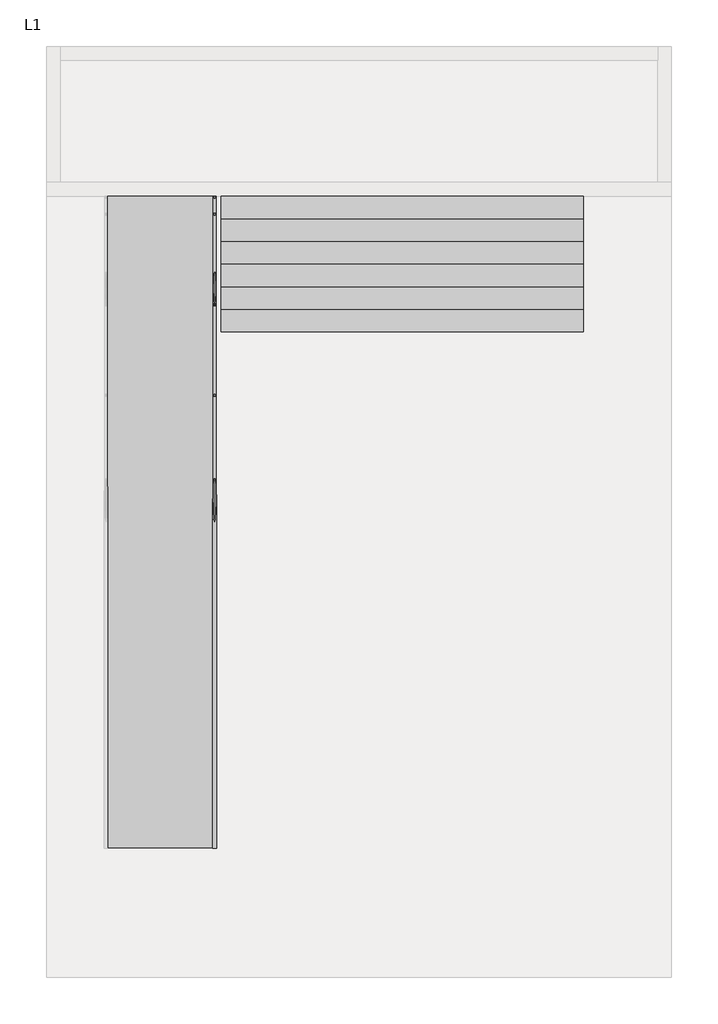
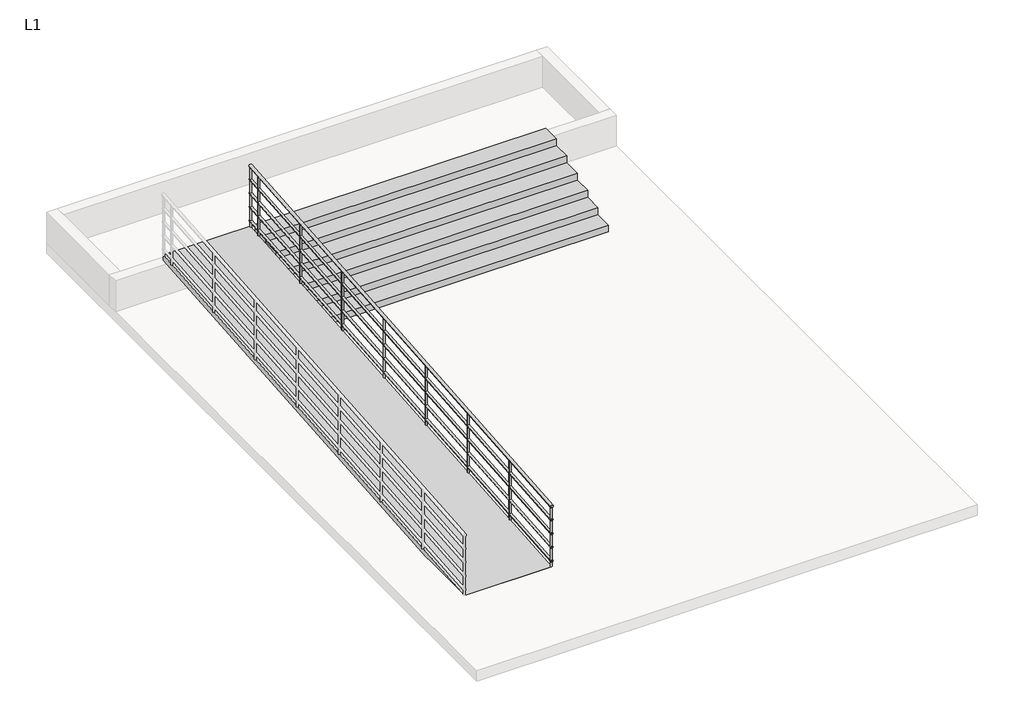
# One storey, part 2 of 2: 1 railing, 1 ramp, 1 stair flight.
"""IFC4 building model written with IfcOpenShell, lengths in millimetres."""

import ifcopenshell
import ifcopenshell.guid

model = None  # the IFC model being written
_history = None  # IfcOwnerHistory: only IFC2X3 demands one
_inside = {}  # id of a spatial element -> (the spatial element, [elements in it])
_under = {}  # id of a project, library or spatial element -> (it, [spatial elements below it])
_declared = {}  # id of a project -> (the project, [libraries it declares])
_typed = {}  # id of a type object -> (the type object, [elements of that type])
_made_of = {}  # id of a material, layer set ... -> (it, [elements and type objects made of it])


def new_model(schema):
    """Start an empty IFC model of exactly this schema.

    Asked for "IFC4X3", IfcOpenShell would pick the latest addendum, in which some entities
    have other attributes; the version numbers below select the first issue.
    IFC2X3 requires an IfcOwnerHistory on every rooted entity: one is made here for all.
    """
    global model, _history
    if schema == "IFC4X3":
        model = ifcopenshell.file(schema_version=(4, 3, 0, 0))
    else:
        model = ifcopenshell.file(schema=schema)
    _inside.clear()
    _under.clear()
    _declared.clear()
    _typed.clear()
    _made_of.clear()
    _history = None
    if model.schema == "IFC2X3":
        org = make("IfcOrganization", Name="unknown")
        user = make(
            "IfcPersonAndOrganization",
            ThePerson=make("IfcPerson", FamilyName="unknown"),
            TheOrganization=org,
        )
        app = make(
            "IfcApplication",
            ApplicationDeveloper=org,
            Version="unknown",
            ApplicationFullName="unknown",
            ApplicationIdentifier="unknown",
        )
        _history = make(
            "IfcOwnerHistory",
            OwningUser=user,
            OwningApplication=app,
            ChangeAction="ADDED",
            CreationDate=0,
        )
    return model


def make(cls, **values):
    """One entity of the class cls with the attributes given. An attribute that is None is left unset."""
    return model.create_entity(
        cls, **{name: value for name, value in values.items() if value is not None}
    )


def rooted(cls, **values):
    """An entity with a GlobalId (a new one), such as an element, a storey or a relation."""
    return make(cls, GlobalId=ifcopenshell.guid.new(), OwnerHistory=_history, **values)


def si_unit(unit_type, name, prefix=None):
    """IfcSIUnit, for example si_unit("LENGTHUNIT", "METRE", prefix="MILLI")."""
    return make("IfcSIUnit", UnitType=unit_type, Prefix=prefix, Name=name)


def assignment(units):
    """IfcUnitAssignment: the units of a project."""
    return None if units is None else make("IfcUnitAssignment", Units=units)


def point(xyz):
    """IfcCartesianPoint."""
    return None if xyz is None else make("IfcCartesianPoint", Coordinates=xyz)


def direction(xyz):
    """IfcDirection."""
    return None if xyz is None else make("IfcDirection", DirectionRatios=xyz)


def frame(location, z_axis=None, x_axis=None):
    """IfcAxis2Placement3D, a coordinate frame: its origin and axes. An axis left out is left unset."""
    return make(
        "IfcAxis2Placement3D",
        Location=point(location),
        Axis=direction(z_axis),
        RefDirection=direction(x_axis),
    )


def origin():
    """The frame at (0, 0, 0) with its axes left unset."""
    return frame((0.0, 0.0, 0.0))


def place(relative_to, where):
    """IfcLocalPlacement: puts the frame where relative to a parent placement (None: the world)."""
    return make(
        "IfcLocalPlacement", PlacementRelTo=relative_to, RelativePlacement=where
    )


def context(
    kind, dimensions, precision=None, world=None, true_north=None, identifier=None
):
    """IfcGeometricRepresentationContext, for example the 3D "Model" context."""
    return make(
        "IfcGeometricRepresentationContext",
        ContextIdentifier=identifier,
        ContextType=kind,
        CoordinateSpaceDimension=dimensions,
        Precision=precision,
        WorldCoordinateSystem=world,
        TrueNorth=true_north,
    )


def project(units=None, contexts=None):
    """IfcProject with its units and contexts."""
    return rooted(
        "IfcProject",
        Name="project",
        RepresentationContexts=contexts,
        UnitsInContext=assignment(units),
    )


def spatial(cls, under=None, at=None, **own):
    """A site, building, storey or space (cls), placed at a placement, below another one or the project."""
    s = rooted(cls, ObjectPlacement=at, **own)
    if under is not None:
        _under.setdefault(under.id(), (under, []))[1].append(s)
    return s


def polyline(points):
    """IfcPolyline through the points."""
    return make("IfcPolyline", Points=[point(p) for p in points])


def ellipse_curve(where, semi_axis1, semi_axis2):
    """IfcEllipse in the frame where."""
    return make(
        "IfcEllipse", Position=where, SemiAxis1=semi_axis1, SemiAxis2=semi_axis2
    )


def outline(outer, holes=None, kind="AREA"):
    """IfcArbitraryClosedProfileDef: a profile drawn as a closed curve; with holes, ...WithVoids."""
    if holes is None:
        return make("IfcArbitraryClosedProfileDef", ProfileType=kind, OuterCurve=outer)
    return make(
        "IfcArbitraryProfileDefWithVoids",
        ProfileType=kind,
        OuterCurve=outer,
        InnerCurves=holes,
    )


def extrude(swept, where, along, depth):
    """IfcExtrudedAreaSolid: the profile swept, set in the frame where, extruded along a direction by depth."""
    return make(
        "IfcExtrudedAreaSolid",
        SweptArea=swept,
        Position=where,
        ExtrudedDirection=direction(along),
        Depth=depth,
    )


def faces_of(points, faces, orient=None, outer=None):
    """IfcFace entities. A face is a list of loops; a loop is a list of indices into points, from 0.

    orient and outer hold one flag for each loop. By default every Orientation is true, the
    first loop of a face is its IfcFaceOuterBound and the others are IfcFaceBound.
    """
    made = []
    for i, loops in enumerate(faces):
        bounds = []
        for j, loop in enumerate(loops):
            is_outer = j == 0 if outer is None else outer[i][j]
            bounds.append(
                make(
                    "IfcFaceOuterBound" if is_outer else "IfcFaceBound",
                    Bound=make("IfcPolyLoop", Polygon=[points[k] for k in loop]),
                    Orientation=True if orient is None else orient[i][j],
                )
            )
        made.append(make("IfcFace", Bounds=bounds))
    return made


def faceted_brep(points, faces, orient=None, outer=None, voids=None):
    """IfcFacetedBrep: a solid bounded by flat faces; with voids (closed shells), ...WithVoids."""
    shared = [point(p) for p in points]
    hull = make("IfcClosedShell", CfsFaces=faces_of(shared, faces, orient, outer))
    if voids is None:
        return make("IfcFacetedBrep", Outer=hull)
    return make(
        "IfcFacetedBrepWithVoids",
        Outer=hull,
        Voids=[
            make(cls, CfsFaces=faces_of(shared, fs, o, b)) for cls, fs, o, b in voids
        ],
    )


def shape(context_of_items, identifier, shape_type, items):
    """IfcShapeRepresentation: the items that make up one representation, for example the "Body"."""
    return make(
        "IfcShapeRepresentation",
        ContextOfItems=context_of_items,
        RepresentationIdentifier=identifier,
        RepresentationType=shape_type,
        Items=items,
    )


def source(mapping_origin, context_of_items, identifier, shape_type, items):
    """IfcRepresentationMap: a shape defined once, which mapped items show again and again."""
    return make(
        "IfcRepresentationMap",
        MappingOrigin=mapping_origin,
        MappedRepresentation=shape(context_of_items, identifier, shape_type, items),
    )


def transform(
    local_origin,
    x_axis=None,
    y_axis=None,
    z_axis=None,
    scale=None,
    scale2=None,
    scale3=None,
    uniform=True,
):
    """IfcCartesianTransformationOperator3D, or its non-uniform kind. x_axis, y_axis, z_axis: its Axis1, 2, 3."""
    if uniform:
        return make(
            "IfcCartesianTransformationOperator3D",
            Axis1=direction(x_axis),
            Axis2=direction(y_axis),
            LocalOrigin=point(local_origin),
            Scale=scale,
            Axis3=direction(z_axis),
        )
    return make(
        "IfcCartesianTransformationOperator3DnonUniform",
        Axis1=direction(x_axis),
        Axis2=direction(y_axis),
        LocalOrigin=point(local_origin),
        Scale=scale,
        Axis3=direction(z_axis),
        Scale2=scale2,
        Scale3=scale3,
    )


def mapped(mapping_source, mapping_target):
    """IfcMappedItem: shows the shape of a source again, moved by a transform."""
    return make(
        "IfcMappedItem", MappingSource=mapping_source, MappingTarget=mapping_target
    )


def made_of(thing, what):
    """Note that an element or type object is made of a material, layer set ...; save() writes the relation."""
    if what is not None:
        _made_of.setdefault(what.id(), (what, []))[1].append(thing)
    return thing


def element(
    cls,
    number,
    at=None,
    inside=None,
    cuts=None,
    type_object=None,
    material=None,
    context=None,
    identifier="Body",
    shape_type=None,
    held_by="IfcProductDefinitionShape",
    body=None,
    shapes=None,
    **own,
):
    """One element of the class cls, such as IfcWall. Its Tag is "e" and its number.

    at: its placement. inside: the storey or other place that contains it. cuts: it is an
    opening in that element (IfcRelVoidsElement). A single representation is given by context,
    identifier, shape_type and body (its items); several are given by shapes. held_by: the class
    of the entity that holds the representations. save() writes the other relations.
    """
    e = rooted(cls, Tag="e%d" % number, ObjectPlacement=at, **own)
    if body is not None:
        shapes = [shape(context, identifier, shape_type, body)]
    if shapes is not None:
        e.Representation = make(held_by, Representations=shapes)
    if inside is not None:
        _inside.setdefault(inside.id(), (inside, []))[1].append(e)
    if cuts is not None:
        rooted(
            "IfcRelVoidsElement", RelatingBuildingElement=cuts, RelatedOpeningElement=e
        )
    if type_object is not None:
        _typed.setdefault(type_object.id(), (type_object, []))[1].append(e)
    return made_of(e, material)


def aggregate(whole, parts):
    """IfcRelAggregates: a whole, such as a stair, and the parts it consists of."""
    return rooted("IfcRelAggregates", RelatingObject=whole, RelatedObjects=parts)


def save(model, path):
    """Write the relations noted so far, then the file.

    IfcRelAggregates (storeys below a building ...), IfcRelContainedInSpatialStructure (elements
    in a storey), IfcRelDefinesByType, IfcRelAssociatesMaterial and IfcRelDeclares: one each for
    every whole, place, type object, material and project.
    """
    for whole, parts in _under.values():
        aggregate(whole, parts)
    for where, things in _inside.values():
        rooted(
            "IfcRelContainedInSpatialStructure",
            RelatedElements=things,
            RelatingStructure=where,
        )
    for kind, things in _typed.values():
        rooted("IfcRelDefinesByType", RelatedObjects=things, RelatingType=kind)
    for what, things in _made_of.values():
        rooted("IfcRelAssociatesMaterial", RelatedObjects=things, RelatingMaterial=what)
    for by, libraries in _declared.values():
        rooted("IfcRelDeclares", RelatingContext=by, RelatedDefinitions=libraries)
    model.write(path)


def plane_surface(at):
    """IfcPlane: the flat surface through the origin of the frame at, square to its z axis."""
    return make("IfcPlane", Position=at)


def cylinder_surface(at, radius):
    """IfcCylindricalSurface: all points at the distance radius from the z axis of the frame at."""
    return make("IfcCylindricalSurface", Position=at, Radius=radius)


def advanced_brep(points, edges, surfaces, faces):
    """IfcAdvancedBrep: a solid bounded by faces that lie on surfaces and meet in shared edges.

    An edge is (start, end): straight between two places in points (the first is 0);
    or (start, end, curve); or (start, end, curve, False) where it runs against its curve.
    A face is (place in surfaces, loops), or (place, loops, False) where it looks against
    its surface's normal. A loop lists edges by number (the first is 1), with a minus sign
    where the edge is run from its end to its start. The first loop is the outer one.
    """
    corners = [point(p) for p in points]
    vertices = [make("IfcVertexPoint", VertexGeometry=c) for c in corners]
    made = []
    for start, end, *more in edges:
        made.append(
            make(
                "IfcEdgeCurve",
                EdgeStart=vertices[start],
                EdgeEnd=vertices[end],
                EdgeGeometry=more[0] if more else make("IfcPolyline", Points=[corners[start], corners[end]]),
                SameSense=more[1] if len(more) > 1 else True,
            )
        )
    hull = []
    for where, loops, *sense in faces:
        bounds = []
        for j, loop in enumerate(loops):
            ring = [make("IfcOrientedEdge", EdgeElement=made[abs(k) - 1], Orientation=k > 0) for k in loop]
            bounds.append(
                make(
                    "IfcFaceOuterBound" if j == 0 else "IfcFaceBound",
                    Bound=make("IfcEdgeLoop", EdgeList=ring),
                    Orientation=True,
                )
            )
        hull.append(make("IfcAdvancedFace", Bounds=bounds, FaceSurface=surfaces[where], SameSense=sense[0] if sense else True))
    return make("IfcAdvancedBrep", Outer=make("IfcClosedShell", CfsFaces=hull))


def ramp_1_51a07ffc(model_context):
    return source(origin(), model_context, "Body", "SweptSolid", [
        extrude(outline(polyline([(-8058.4292912, 0.0), (-858.4292912, 600.0), (-858.4292912, 524.7400339), (-8058.4292912, -75.2599661), (-8058.4292912, 0.0)])), frame((-599.8488078, 0.0, 0.0), z_axis=(1.0, 0.0, 0.0), x_axis=(0.0, 1.0, 0.0)), (0.0, 0.0, 1.0), 1200.0),
    ])


model = new_model("IFC4")

# Units and contexts
model_context = context("Model", 3, world=origin())
ifc_project = project(units=[si_unit("LENGTHUNIT", "METRE", prefix="MILLI")], contexts=[model_context])

# Site, building, storey
site = spatial("IfcSite", under=ifc_project)
building = spatial("IfcBuilding", under=site)
storey = spatial("IfcBuildingStorey", under=building, Name="L1", Elevation=0.0)

# Railing
placement = place(None, origin())
element("IfcRailing", 1, ObjectType="900mm Pipe", at=placement, inside=storey, context=model_context, shape_type="AdvancedBrep", body=[
    advanced_brep(
    [(620.1511922, -8058.4292912, 879.9306757), (580.1511922, -8058.4292912, 879.9306757), (620.1511922, -858.4292912, 1479.9306757), (580.1511922, -858.4292912, 1479.9306757)],
    [
        (0, 1, ellipse_curve(frame((600.1511922, -8058.4292912, 879.9306757), z_axis=(0.0, -1.0, 0.0), x_axis=(0.0, 0.0, -1.0)), 20.0693243, 20.0)),
        (1, 0, ellipse_curve(frame((600.1511922, -8058.4292912, 879.9306757), z_axis=(0.0, -1.0, 0.0), x_axis=(0.0, 0.0, -1.0)), 20.0693243, 20.0)),
        (2, 3, ellipse_curve(frame((600.1511922, -858.4292912, 1479.9306757), z_axis=(0.0, 1.0, 0.0), x_axis=(0.0, 0.0, -1.0)), 20.0693243, 20.0)),
        (3, 2, ellipse_curve(frame((600.1511922, -858.4292912, 1479.9306757), z_axis=(0.0, 1.0, 0.0), x_axis=(0.0, 0.0, -1.0)), 20.0693243, 20.0)),
        (0, 2),
        (3, 1),
    ],
    [
        plane_surface(frame((600.1511922, -8058.4292912, 900.0), z_axis=(0.0, -1.0, 0.0), x_axis=(0.0, 0.0, 1.0))),
        plane_surface(frame((600.1511922, -858.4292912, 1500.0), z_axis=(0.0, 1.0, 0.0), x_axis=(0.0, 0.0, 1.0))),
        cylinder_surface(frame((600.1511922, -8056.7683816, 880.0690848), z_axis=(0.0, -0.9965457582448797, -0.08304547985373999), x_axis=(-1.0, 0.0, 0.0)), 20.0),
    ],
    [
        (0, [[1, 2]]),
        (1, [[3, 4]]),
        (2, [[-1, 5, -4, 6]]),
        (2, [[-2, -6, -3, -5]]),
    ],
),
    advanced_brep(
    [(615.1511922, -8058.4292912, 684.9480068), (585.1511922, -8058.4292912, 684.9480068), (615.1511922, -858.4292912, 1284.9480068), (585.1511922, -858.4292912, 1284.9480068)],
    [
        (0, 1, ellipse_curve(frame((600.1511922, -8058.4292912, 684.9480068), z_axis=(0.0, -1.0, 0.0), x_axis=(0.0, 0.0, -0.9999999999999999)), 15.0519932, 15.0)),
        (1, 0, ellipse_curve(frame((600.1511922, -8058.4292912, 684.9480068), z_axis=(0.0, -1.0, 0.0), x_axis=(0.0, 0.0, -0.9999999999999999)), 15.0519932, 15.0)),
        (2, 3, ellipse_curve(frame((600.1511922, -858.4292912, 1284.9480068), z_axis=(0.0, 1.0, 0.0), x_axis=(0.0, 0.0, -0.9999999999999999)), 15.0519932, 15.0)),
        (3, 2, ellipse_curve(frame((600.1511922, -858.4292912, 1284.9480068), z_axis=(0.0, 1.0, 0.0), x_axis=(0.0, 0.0, -0.9999999999999999)), 15.0519932, 15.0)),
        (0, 2),
        (3, 1),
    ],
    [
        plane_surface(frame((600.1511922, -8058.4292912, 700.0), z_axis=(0.0, -1.0, 0.0), x_axis=(0.0, 0.0, 1.0))),
        plane_surface(frame((600.1511922, -858.4292912, 1300.0), z_axis=(0.0, 1.0, 0.0), x_axis=(0.0, 0.0, 1.0))),
        cylinder_surface(frame((600.1511922, -8057.183609, 685.0518136), z_axis=(0.0, -0.9965457582448797, -0.08304547985373997), x_axis=(-1.0, 0.0, 0.0)), 15.0),
    ],
    [
        (0, [[1, 2]]),
        (1, [[3, 4]]),
        (2, [[-1, 5, -4, 6]]),
        (2, [[-2, -6, -3, -5]]),
    ],
),
    advanced_brep(
    [(615.1511922, -8058.4292912, 484.9480068), (585.1511922, -8058.4292912, 484.9480068), (615.1511922, -858.4292912, 1084.9480068), (585.1511922, -858.4292912, 1084.9480068)],
    [
        (0, 1, ellipse_curve(frame((600.1511922, -8058.4292912, 484.9480068), z_axis=(0.0, -1.0, 0.0), x_axis=(0.0, 0.0, -0.9999999999999999)), 15.0519932, 15.0)),
        (1, 0, ellipse_curve(frame((600.1511922, -8058.4292912, 484.9480068), z_axis=(0.0, -1.0, 0.0), x_axis=(0.0, 0.0, -0.9999999999999999)), 15.0519932, 15.0)),
        (2, 3, ellipse_curve(frame((600.1511922, -858.4292912, 1084.9480068), z_axis=(0.0, 1.0, 0.0), x_axis=(0.0, 0.0, -0.9999999999999999)), 15.0519932, 15.0)),
        (3, 2, ellipse_curve(frame((600.1511922, -858.4292912, 1084.9480068), z_axis=(0.0, 1.0, 0.0), x_axis=(0.0, 0.0, -0.9999999999999999)), 15.0519932, 15.0)),
        (0, 2),
        (3, 1),
    ],
    [
        plane_surface(frame((600.1511922, -8058.4292912, 500.0), z_axis=(0.0, -1.0, 0.0), x_axis=(0.0, 0.0, 1.0))),
        plane_surface(frame((600.1511922, -858.4292912, 1100.0), z_axis=(0.0, 1.0, 0.0), x_axis=(0.0, 0.0, 1.0))),
        cylinder_surface(frame((600.1511922, -8057.183609, 485.0518136), z_axis=(0.0, -0.9965457582448797, -0.08304547985373997), x_axis=(-1.0, 0.0, 0.0)), 15.0),
    ],
    [
        (0, [[1, 2]]),
        (1, [[3, 4]]),
        (2, [[-1, 5, -4, 6]]),
        (2, [[-2, -6, -3, -5]]),
    ],
),
    advanced_brep(
    [(615.1511922, -8058.4292912, 284.9480068), (585.1511922, -8058.4292912, 284.9480068), (615.1511922, -858.4292912, 884.9480068), (585.1511922, -858.4292912, 884.9480068)],
    [
        (0, 1, ellipse_curve(frame((600.1511922, -8058.4292912, 284.9480068), z_axis=(0.0, -1.0, 0.0), x_axis=(0.0, 0.0, -0.9999999999999999)), 15.0519932, 15.0)),
        (1, 0, ellipse_curve(frame((600.1511922, -8058.4292912, 284.9480068), z_axis=(0.0, -1.0, 0.0), x_axis=(0.0, 0.0, -0.9999999999999999)), 15.0519932, 15.0)),
        (2, 3, ellipse_curve(frame((600.1511922, -858.4292912, 884.9480068), z_axis=(0.0, 1.0, 0.0), x_axis=(0.0, 0.0, -0.9999999999999999)), 15.0519932, 15.0)),
        (3, 2, ellipse_curve(frame((600.1511922, -858.4292912, 884.9480068), z_axis=(0.0, 1.0, 0.0), x_axis=(0.0, 0.0, -0.9999999999999999)), 15.0519932, 15.0)),
        (0, 2),
        (3, 1),
    ],
    [
        plane_surface(frame((600.1511922, -8058.4292912, 300.0), z_axis=(0.0, -1.0, 0.0), x_axis=(0.0, 0.0, 1.0))),
        plane_surface(frame((600.1511922, -858.4292912, 900.0), z_axis=(0.0, 1.0, 0.0), x_axis=(0.0, 0.0, 1.0))),
        cylinder_surface(frame((600.1511922, -8057.183609, 285.0518136), z_axis=(0.0, -0.9965457582448797, -0.08304547985373997), x_axis=(-1.0, 0.0, 0.0)), 15.0),
    ],
    [
        (0, [[1, 2]]),
        (1, [[3, 4]]),
        (2, [[-1, 5, -4, 6]]),
        (2, [[-2, -6, -3, -5]]),
    ],
),
    advanced_brep(
    [(615.1511922, -8058.4292912, 84.9480068), (585.1511922, -8058.4292912, 84.9480068), (615.1511922, -858.4292912, 684.9480068), (585.1511922, -858.4292912, 684.9480068)],
    [
        (0, 1, ellipse_curve(frame((600.1511922, -8058.4292912, 84.9480068), z_axis=(0.0, -1.0, 0.0), x_axis=(0.0, 0.0, -0.9999999999999999)), 15.0519932, 15.0)),
        (1, 0, ellipse_curve(frame((600.1511922, -8058.4292912, 84.9480068), z_axis=(0.0, -1.0, 0.0), x_axis=(0.0, 0.0, -0.9999999999999999)), 15.0519932, 15.0)),
        (2, 3, ellipse_curve(frame((600.1511922, -858.4292912, 684.9480068), z_axis=(0.0, 1.0, 0.0), x_axis=(0.0, 0.0, -0.9999999999999999)), 15.0519932, 15.0)),
        (3, 2, ellipse_curve(frame((600.1511922, -858.4292912, 684.9480068), z_axis=(0.0, 1.0, 0.0), x_axis=(0.0, 0.0, -0.9999999999999999)), 15.0519932, 15.0)),
        (0, 2),
        (3, 1),
    ],
    [
        plane_surface(frame((600.1511922, -8058.4292912, 100.0), z_axis=(0.0, -1.0, 0.0), x_axis=(0.0, 0.0, 1.0))),
        plane_surface(frame((600.1511922, -858.4292912, 700.0), z_axis=(0.0, 1.0, 0.0), x_axis=(0.0, 0.0, 1.0))),
        cylinder_surface(frame((600.1511922, -8057.183609, 85.0518136), z_axis=(0.0, -0.9965457582448797, -0.08304547985373997), x_axis=(-1.0, 0.0, 0.0)), 15.0),
    ],
    [
        (0, [[1, 2]]),
        (1, [[3, 4]]),
        (2, [[-1, 5, -4, 6]]),
        (2, [[-2, -6, -3, -5]]),
    ],
),
    advanced_brep(
    [(587.6511922, -1058.4292912, 1443.1946847), (612.6511922, -1058.4292912, 1443.1946847), (612.6511922, -1058.4292912, 583.3333333), (587.6511922, -1058.4292912, 583.3333333)],
    [
        (0, 1, ellipse_curve(frame((600.1511922, -1058.4292912, 1443.1946847), z_axis=(0.0, 0.08304547985373997, -0.9965457582448797), x_axis=(0.0, 0.9965457582448797, 0.0830454798537388)), 12.5433277, 12.5)),
        (1, 2),
        (2, 3, ellipse_curve(frame((600.1511922, -1058.4292912, 583.3333333), z_axis=(0.0, -0.08304547985373995, 0.9965457582448797), x_axis=(0.0, 0.9965457582448798, 0.08304547985373882)), 12.5433277, 12.5)),
        (3, 0),
        (3, 2, ellipse_curve(frame((600.1511922, -1058.4292912, 583.3333333), z_axis=(0.0, -0.08304547985373995, 0.9965457582448797), x_axis=(0.0, 0.9965457582448798, 0.08304547985373882)), 12.5433277, 12.5)),
        (1, 0, ellipse_curve(frame((600.1511922, -1058.4292912, 1443.1946847), z_axis=(0.0, 0.08304547985373997, -0.9965457582448797), x_axis=(0.0, 0.9965457582448797, 0.0830454798537388)), 12.5433277, 12.5)),
    ],
    [
        cylinder_surface(frame((600.1511922, -1058.4292912, 483.3333333), z_axis=(0.0, 0.0, 1.0), x_axis=(1.0, 0.0, 0.0)), 12.5),
        plane_surface(frame((625.1511922, -1033.4292912, 1445.2780181), z_axis=(0.0, -0.08304547985373997, 0.9965457582448797), x_axis=(-1.0, 0.0, 0.0))),
        plane_surface(frame((625.1511922, -1083.4292912, 581.25), z_axis=(0.0, 0.08304547985373995, -0.9965457582448797), x_axis=(-1.0, 0.0, 0.0))),
    ],
    [
        (0, [[1, 2, 3, 4]]),
        (0, [[5, -2, 6, -4]]),
        (1, [[-6, -1]]),
        (2, [[-5, -3]]),
    ],
),
    advanced_brep(
    [(587.6511922, -2058.4292912, 1359.8613514), (612.6511922, -2058.4292912, 1359.8613514), (612.6511922, -2058.4292912, 500.0), (587.6511922, -2058.4292912, 500.0)],
    [
        (0, 1, ellipse_curve(frame((600.1511922, -2058.4292912, 1359.8613514), z_axis=(0.0, 0.08304547985373997, -0.9965457582448797), x_axis=(0.0, 0.9965457582448797, 0.0830454798537388)), 12.5433277, 12.5)),
        (1, 2),
        (2, 3, ellipse_curve(frame((600.1511922, -2058.4292912, 500.0), z_axis=(0.0, -0.08304547985373995, 0.9965457582448797), x_axis=(0.0, 0.9965457582448798, 0.08304547985373882)), 12.5433277, 12.5)),
        (3, 0),
        (3, 2, ellipse_curve(frame((600.1511922, -2058.4292912, 500.0), z_axis=(0.0, -0.08304547985373995, 0.9965457582448797), x_axis=(0.0, 0.9965457582448798, 0.08304547985373882)), 12.5433277, 12.5)),
        (1, 0, ellipse_curve(frame((600.1511922, -2058.4292912, 1359.8613514), z_axis=(0.0, 0.08304547985373997, -0.9965457582448797), x_axis=(0.0, 0.9965457582448797, 0.0830454798537388)), 12.5433277, 12.5)),
    ],
    [
        cylinder_surface(frame((600.1511922, -2058.4292912, 400.0), z_axis=(0.0, 0.0, 1.0), x_axis=(1.0, 0.0, 0.0)), 12.5),
        plane_surface(frame((625.1511922, -2033.4292912, 1361.9446847), z_axis=(0.0, -0.08304547985373997, 0.9965457582448797), x_axis=(-1.0, 0.0, 0.0))),
        plane_surface(frame((625.1511922, -2083.4292912, 497.9166667), z_axis=(0.0, 0.08304547985373995, -0.9965457582448797), x_axis=(-1.0, 0.0, 0.0))),
    ],
    [
        (0, [[1, 2, 3, 4]]),
        (0, [[5, -2, 6, -4]]),
        (1, [[-6, -1]]),
        (2, [[-5, -3]]),
    ],
),
    advanced_brep(
    [(587.6511922, -3058.4292912, 1276.5280181), (612.6511922, -3058.4292912, 1276.5280181), (612.6511922, -3058.4292912, 416.6666667), (587.6511922, -3058.4292912, 416.6666667)],
    [
        (0, 1, ellipse_curve(frame((600.1511922, -3058.4292912, 1276.5280181), z_axis=(0.0, 0.08304547985373997, -0.9965457582448797), x_axis=(0.0, 0.9965457582448797, 0.0830454798537388)), 12.5433277, 12.5)),
        (1, 2),
        (2, 3, ellipse_curve(frame((600.1511922, -3058.4292912, 416.6666667), z_axis=(0.0, -0.08304547985373995, 0.9965457582448797), x_axis=(0.0, 0.9965457582448798, 0.08304547985373882)), 12.5433277, 12.5)),
        (3, 0),
        (3, 2, ellipse_curve(frame((600.1511922, -3058.4292912, 416.6666667), z_axis=(0.0, -0.08304547985373995, 0.9965457582448797), x_axis=(0.0, 0.9965457582448798, 0.08304547985373882)), 12.5433277, 12.5)),
        (1, 0, ellipse_curve(frame((600.1511922, -3058.4292912, 1276.5280181), z_axis=(0.0, 0.08304547985373997, -0.9965457582448797), x_axis=(0.0, 0.9965457582448797, 0.0830454798537388)), 12.5433277, 12.5)),
    ],
    [
        cylinder_surface(frame((600.1511922, -3058.4292912, 316.6666667), z_axis=(0.0, 0.0, 1.0), x_axis=(1.0, 0.0, 0.0)), 12.5),
        plane_surface(frame((625.1511922, -3033.4292912, 1278.6113514), z_axis=(0.0, -0.08304547985373997, 0.9965457582448797), x_axis=(-1.0, 0.0, 0.0))),
        plane_surface(frame((625.1511922, -3083.4292912, 414.5833333), z_axis=(0.0, 0.08304547985373995, -0.9965457582448797), x_axis=(-1.0, 0.0, 0.0))),
    ],
    [
        (0, [[1, 2, 3, 4]]),
        (0, [[5, -2, 6, -4]]),
        (1, [[-6, -1]]),
        (2, [[-5, -3]]),
    ],
),
    advanced_brep(
    [(587.6511922, -4058.4292912, 1193.1946847), (612.6511922, -4058.4292912, 1193.1946847), (612.6511922, -4058.4292912, 333.3333333), (587.6511922, -4058.4292912, 333.3333333)],
    [
        (0, 1, ellipse_curve(frame((600.1511922, -4058.4292912, 1193.1946847), z_axis=(0.0, 0.08304547985373997, -0.9965457582448797), x_axis=(0.0, 0.9965457582448797, 0.0830454798537388)), 12.5433277, 12.5)),
        (1, 2),
        (2, 3, ellipse_curve(frame((600.1511922, -4058.4292912, 333.3333333), z_axis=(0.0, -0.08304547985373995, 0.9965457582448797), x_axis=(0.0, 0.9965457582448798, 0.08304547985373882)), 12.5433277, 12.5)),
        (3, 0),
        (3, 2, ellipse_curve(frame((600.1511922, -4058.4292912, 333.3333333), z_axis=(0.0, -0.08304547985373995, 0.9965457582448797), x_axis=(0.0, 0.9965457582448798, 0.08304547985373882)), 12.5433277, 12.5)),
        (1, 0, ellipse_curve(frame((600.1511922, -4058.4292912, 1193.1946847), z_axis=(0.0, 0.08304547985373997, -0.9965457582448797), x_axis=(0.0, 0.9965457582448797, 0.0830454798537388)), 12.5433277, 12.5)),
    ],
    [
        cylinder_surface(frame((600.1511922, -4058.4292912, 233.3333333), z_axis=(0.0, 0.0, 1.0), x_axis=(1.0, 0.0, 0.0)), 12.5),
        plane_surface(frame((625.1511922, -4033.4292912, 1195.2780181), z_axis=(0.0, -0.08304547985373997, 0.9965457582448797), x_axis=(-1.0, 0.0, 0.0))),
        plane_surface(frame((625.1511922, -4083.4292912, 331.25), z_axis=(0.0, 0.08304547985373995, -0.9965457582448797), x_axis=(-1.0, 0.0, 0.0))),
    ],
    [
        (0, [[1, 2, 3, 4]]),
        (0, [[5, -2, 6, -4]]),
        (1, [[-6, -1]]),
        (2, [[-5, -3]]),
    ],
),
    advanced_brep(
    [(587.6511922, -5058.4292912, 1109.8613514), (612.6511922, -5058.4292912, 1109.8613514), (612.6511922, -5058.4292912, 250.0), (587.6511922, -5058.4292912, 250.0)],
    [
        (0, 1, ellipse_curve(frame((600.1511922, -5058.4292912, 1109.8613514), z_axis=(0.0, 0.08304547985373997, -0.9965457582448797), x_axis=(0.0, 0.9965457582448797, 0.0830454798537388)), 12.5433277, 12.5)),
        (1, 2),
        (2, 3, ellipse_curve(frame((600.1511922, -5058.4292912, 250.0), z_axis=(0.0, -0.08304547985373995, 0.9965457582448797), x_axis=(0.0, 0.9965457582448798, 0.08304547985373882)), 12.5433277, 12.5)),
        (3, 0),
        (3, 2, ellipse_curve(frame((600.1511922, -5058.4292912, 250.0), z_axis=(0.0, -0.08304547985373995, 0.9965457582448797), x_axis=(0.0, 0.9965457582448798, 0.08304547985373882)), 12.5433277, 12.5)),
        (1, 0, ellipse_curve(frame((600.1511922, -5058.4292912, 1109.8613514), z_axis=(0.0, 0.08304547985373997, -0.9965457582448797), x_axis=(0.0, 0.9965457582448797, 0.0830454798537388)), 12.5433277, 12.5)),
    ],
    [
        cylinder_surface(frame((600.1511922, -5058.4292912, 150.0), z_axis=(0.0, 0.0, 1.0), x_axis=(1.0, 0.0, 0.0)), 12.5),
        plane_surface(frame((625.1511922, -5033.4292912, 1111.9446847), z_axis=(0.0, -0.08304547985373997, 0.9965457582448797), x_axis=(-1.0, 0.0, 0.0))),
        plane_surface(frame((625.1511922, -5083.4292912, 247.9166667), z_axis=(0.0, 0.08304547985373995, -0.9965457582448797), x_axis=(-1.0, 0.0, 0.0))),
    ],
    [
        (0, [[1, 2, 3, 4]]),
        (0, [[5, -2, 6, -4]]),
        (1, [[-6, -1]]),
        (2, [[-5, -3]]),
    ],
),
    advanced_brep(
    [(587.6511922, -6058.4292912, 1026.5280181), (612.6511922, -6058.4292912, 1026.5280181), (612.6511922, -6058.4292912, 166.6666667), (587.6511922, -6058.4292912, 166.6666667)],
    [
        (0, 1, ellipse_curve(frame((600.1511922, -6058.4292912, 1026.5280181), z_axis=(0.0, 0.08304547985373997, -0.9965457582448797), x_axis=(0.0, 0.9965457582448797, 0.0830454798537388)), 12.5433277, 12.5)),
        (1, 2),
        (2, 3, ellipse_curve(frame((600.1511922, -6058.4292912, 166.6666667), z_axis=(0.0, -0.08304547985373995, 0.9965457582448797), x_axis=(0.0, 0.9965457582448798, 0.08304547985373882)), 12.5433277, 12.5)),
        (3, 0),
        (3, 2, ellipse_curve(frame((600.1511922, -6058.4292912, 166.6666667), z_axis=(0.0, -0.08304547985373995, 0.9965457582448797), x_axis=(0.0, 0.9965457582448798, 0.08304547985373882)), 12.5433277, 12.5)),
        (1, 0, ellipse_curve(frame((600.1511922, -6058.4292912, 1026.5280181), z_axis=(0.0, 0.08304547985373997, -0.9965457582448797), x_axis=(0.0, 0.9965457582448797, 0.0830454798537388)), 12.5433277, 12.5)),
    ],
    [
        cylinder_surface(frame((600.1511922, -6058.4292912, 66.6666667), z_axis=(0.0, 0.0, 1.0), x_axis=(1.0, 0.0, 0.0)), 12.5),
        plane_surface(frame((625.1511922, -6033.4292912, 1028.6113514), z_axis=(0.0, -0.08304547985373997, 0.9965457582448797), x_axis=(-1.0, 0.0, 0.0))),
        plane_surface(frame((625.1511922, -6083.4292912, 164.5833333), z_axis=(0.0, 0.08304547985373995, -0.9965457582448797), x_axis=(-1.0, 0.0, 0.0))),
    ],
    [
        (0, [[1, 2, 3, 4]]),
        (0, [[5, -2, 6, -4]]),
        (1, [[-6, -1]]),
        (2, [[-5, -3]]),
    ],
),
    advanced_brep(
    [(587.6511922, -7058.4292912, 943.1946847), (612.6511922, -7058.4292912, 943.1946847), (612.6511922, -7058.4292912, 83.3333333), (587.6511922, -7058.4292912, 83.3333333)],
    [
        (0, 1, ellipse_curve(frame((600.1511922, -7058.4292912, 943.1946847), z_axis=(0.0, 0.08304547985373997, -0.9965457582448797), x_axis=(0.0, 0.9965457582448797, 0.0830454798537388)), 12.5433277, 12.5)),
        (1, 2),
        (2, 3, ellipse_curve(frame((600.1511922, -7058.4292912, 83.3333333), z_axis=(0.0, -0.08304547985373995, 0.9965457582448797), x_axis=(0.0, 0.9965457582448798, 0.08304547985373882)), 12.5433277, 12.5)),
        (3, 0),
        (3, 2, ellipse_curve(frame((600.1511922, -7058.4292912, 83.3333333), z_axis=(0.0, -0.08304547985373995, 0.9965457582448797), x_axis=(0.0, 0.9965457582448798, 0.08304547985373882)), 12.5433277, 12.5)),
        (1, 0, ellipse_curve(frame((600.1511922, -7058.4292912, 943.1946847), z_axis=(0.0, 0.08304547985373997, -0.9965457582448797), x_axis=(0.0, 0.9965457582448797, 0.0830454798537388)), 12.5433277, 12.5)),
    ],
    [
        cylinder_surface(frame((600.1511922, -7058.4292912, -16.6666667), z_axis=(0.0, 0.0, 1.0), x_axis=(1.0, 0.0, 0.0)), 12.5),
        plane_surface(frame((625.1511922, -7033.4292912, 945.2780181), z_axis=(0.0, -0.08304547985373997, 0.9965457582448797), x_axis=(-1.0, 0.0, 0.0))),
        plane_surface(frame((625.1511922, -7083.4292912, 81.25), z_axis=(0.0, 0.08304547985373995, -0.9965457582448797), x_axis=(-1.0, 0.0, 0.0))),
    ],
    [
        (0, [[1, 2, 3, 4]]),
        (0, [[5, -2, 6, -4]]),
        (1, [[-6, -1]]),
        (2, [[-5, -3]]),
    ],
),
    advanced_brep(
    [(587.6511922, -870.9292912, 1458.8196847), (612.6511922, -870.9292912, 1458.8196847), (612.6511922, -870.9292912, 598.9583333), (587.6511922, -870.9292912, 598.9583333)],
    [
        (0, 1, ellipse_curve(frame((600.1511922, -870.9292912, 1458.8196847), z_axis=(0.0, 0.08304547985373997, -0.9965457582448797), x_axis=(0.0, 0.9965457582448797, 0.0830454798537388)), 12.5433277, 12.5)),
        (1, 2),
        (2, 3, ellipse_curve(frame((600.1511922, -870.9292912, 598.9583333), z_axis=(0.0, -0.08304547985373995, 0.9965457582448797), x_axis=(0.0, 0.9965457582448798, 0.08304547985373882)), 12.5433277, 12.5)),
        (3, 0),
        (3, 2, ellipse_curve(frame((600.1511922, -870.9292912, 598.9583333), z_axis=(0.0, -0.08304547985373995, 0.9965457582448797), x_axis=(0.0, 0.9965457582448798, 0.08304547985373882)), 12.5433277, 12.5)),
        (1, 0, ellipse_curve(frame((600.1511922, -870.9292912, 1458.8196847), z_axis=(0.0, 0.08304547985373997, -0.9965457582448797), x_axis=(0.0, 0.9965457582448797, 0.0830454798537388)), 12.5433277, 12.5)),
    ],
    [
        cylinder_surface(frame((600.1511922, -870.9292912, 498.9583333), z_axis=(0.0, 0.0, 1.0), x_axis=(1.0, 0.0, 0.0)), 12.5),
        plane_surface(frame((625.1511922, -845.9292912, 1460.9030181), z_axis=(0.0, -0.08304547985373997, 0.9965457582448797), x_axis=(-1.0, 0.0, 0.0))),
        plane_surface(frame((625.1511922, -895.9292912, 596.875), z_axis=(0.0, 0.08304547985373995, -0.9965457582448797), x_axis=(-1.0, 0.0, 0.0))),
    ],
    [
        (0, [[1, 2, 3, 4]]),
        (0, [[5, -2, 6, -4]]),
        (1, [[-6, -1]]),
        (2, [[-5, -3]]),
    ],
),
    advanced_brep(
    [(587.6511922, -8045.9292912, 860.9030181), (612.6511922, -8045.9292912, 860.9030181), (612.6511922, -8045.9292912, 1.0416667), (587.6511922, -8045.9292912, 1.0416667)],
    [
        (0, 1, ellipse_curve(frame((600.1511922, -8045.9292912, 860.9030181), z_axis=(0.0, 0.08304547985373997, -0.9965457582448797), x_axis=(0.0, 0.9965457582448797, 0.0830454798537388)), 12.5433277, 12.5)),
        (1, 2),
        (2, 3, ellipse_curve(frame((600.1511922, -8045.9292912, 1.0416667), z_axis=(0.0, -0.08304547985373995, 0.9965457582448797), x_axis=(0.0, 0.9965457582448798, 0.08304547985373882)), 12.5433277, 12.5)),
        (3, 0),
        (3, 2, ellipse_curve(frame((600.1511922, -8045.9292912, 1.0416667), z_axis=(0.0, -0.08304547985373995, 0.9965457582448797), x_axis=(0.0, 0.9965457582448798, 0.08304547985373882)), 12.5433277, 12.5)),
        (1, 0, ellipse_curve(frame((600.1511922, -8045.9292912, 860.9030181), z_axis=(0.0, 0.08304547985373997, -0.9965457582448797), x_axis=(0.0, 0.9965457582448797, 0.0830454798537388)), 12.5433277, 12.5)),
    ],
    [
        cylinder_surface(frame((600.1511922, -8045.9292912, -98.9583333), z_axis=(0.0, 0.0, 1.0), x_axis=(1.0, 0.0, 0.0)), 12.5),
        plane_surface(frame((625.1511922, -8020.9292912, 862.9863514), z_axis=(0.0, -0.08304547985373997, 0.9965457582448797), x_axis=(-1.0, 0.0, 0.0))),
        plane_surface(frame((625.1511922, -8070.9292912, -1.0416667), z_axis=(0.0, 0.08304547985373995, -0.9965457582448797), x_axis=(-1.0, 0.0, 0.0))),
    ],
    [
        (0, [[1, 2, 3, 4]]),
        (0, [[5, -2, 6, -4]]),
        (1, [[-6, -1]]),
        (2, [[-5, -3]]),
    ],
),
])

# Ramp
ramp_1_shape = ramp_1_51a07ffc(model_context)
element("IfcRamp", 2, ObjectType="Ramp 1", at=placement, inside=storey, context=model_context, shape_type="MappedRepresentation", body=[
    mapped(ramp_1_shape, transform((0.0, 0.0, 0.0), x_axis=(1.0, 0.0, 0.0), y_axis=(0.0, 1.0, 0.0), z_axis=(0.0, 0.0, 1.0))),
])

# Stair flight
element("IfcStairFlight", 3, ObjectType="M_Monolithic Run", at=placement, inside=storey, context=model_context, shape_type="Brep", body=[
    faceted_brep([(670.1511922, -2108.4292912, 100.0), (670.1511922, -2358.4292912, 100.0), (4670.1511922, -2358.4292912, 100.0), (4670.1511922, -2108.4292912, 100.0), (670.1511922, -2108.4292912, 0.0), (670.1511922, -2358.4292912, 0.0), (4670.1511922, -2358.4292912, 0.0), (4670.1511922, -2108.4292912, 0.0), (670.1511922, -1858.4292912, 200.0), (670.1511922, -2108.4292912, 200.0), (4670.1511922, -2108.4292912, 200.0), (4670.1511922, -1858.4292912, 200.0), (670.1511922, -1858.4292912, 38.4450558), (670.1511922, -1954.5419306, 0.0), (4670.1511922, -1954.5419306, 0.0), (4670.1511922, -1858.4292912, 38.4450558), (670.1511922, -1608.4292912, 300.0), (670.1511922, -1858.4292912, 300.0), (4670.1511922, -1858.4292912, 300.0), (4670.1511922, -1608.4292912, 300.0), (670.1511922, -1608.4292912, 138.4450558), (4670.1511922, -1608.4292912, 138.4450558), (670.1511922, -1358.4292912, 400.0), (670.1511922, -1608.4292912, 400.0), (4670.1511922, -1608.4292912, 400.0), (4670.1511922, -1358.4292912, 400.0), (670.1511922, -1358.4292912, 238.4450558), (4670.1511922, -1358.4292912, 238.4450558), (670.1511922, -1108.4292912, 500.0), (670.1511922, -1358.4292912, 500.0), (4670.1511922, -1358.4292912, 500.0), (4670.1511922, -1108.4292912, 500.0), (670.1511922, -1108.4292912, 338.4450558), (4670.1511922, -1108.4292912, 338.4450558), (670.1511922, -858.4292912, 600.0), (670.1511922, -1108.4292912, 600.0), (4670.1511922, -1108.4292912, 600.0), (4670.1511922, -858.4292912, 600.0), (670.1511922, -858.4292912, 438.4450558), (4670.1511922, -858.4292912, 438.4450558)], [[[0, 1, 2, 3]], [[1, 0, 4, 5]], [[2, 1, 5, 6]], [[3, 2, 6, 7]], [[8, 9, 10, 11]], [[4, 0, 9, 8, 12, 13]], [[0, 3, 10, 9]], [[3, 7, 14, 15, 11, 10]], [[16, 17, 18, 19]], [[17, 16, 20, 12, 8]], [[8, 11, 18, 17]], [[19, 18, 11, 15, 21]], [[22, 23, 24, 25]], [[23, 22, 26, 20, 16]], [[16, 19, 24, 23]], [[25, 24, 19, 21, 27]], [[28, 29, 30, 31]], [[29, 28, 32, 26, 22]], [[22, 25, 30, 29]], [[31, 30, 25, 27, 33]], [[34, 35, 36, 37]], [[35, 34, 38, 32, 28]], [[28, 31, 36, 35]], [[37, 36, 31, 33, 39]], [[34, 37, 39, 38]], [[5, 4, 13, 14, 7, 6]], [[14, 13, 12, 20, 26, 32, 38, 39, 33, 27, 21, 15]]]),
])

save(model, "model.ifc")

# Revit data of these elements
# Type "900mm Pipe"
#   built-in parameter 1008612 = 0.019685 (stored number, unit not read)
#   built-in parameter 1008611 = 0.0984252 (stored number, unit not read)
#   built-in parameter 1008609 = 3.28084 (stored number, unit not read)
#   built-in parameter 1008604 = 0.19685 (stored number, unit not read)
#   built-in parameter 1008603 = 0.164042 (stored number, unit not read)
#   Railing Height = 900 mm
#   built-in parameter 1008630 = 2
#   built-in parameter 1008610 = 1
#   built-in parameter 1008605 = 1
#   built-in parameter 1008618 = M_Baluster - Round : 25mm
# Type "Ramp 1"
#   built-in parameter 1008304 = 0.246063 (stored number, unit not read)
#   built-in parameter 1008303 = 30 (stored number, unit not read)
#   built-in parameter 1008301 = 12 (stored number, unit not read)
#   Function = 0
# Element 1 (IfcRailing, "900mm Pipe")
#   Phase Created = New Construction
# Element 2 (IfcRamp, "Ramp 1")
#   built-in parameter 1007275 = "DN"
#   built-in parameter 1007272 = "UP"
#   Width = 1200 mm
#   built-in parameter 1007276 = 1
#   built-in parameter 1007274 = 1
#   built-in parameter 1007273 = 1
#   built-in parameter 1007271 = 1
#   Phase Created = New Construction
# Element 3 (IfcStairFlight, "M_Monolithic Run")
#   Phase Created = New Construction
